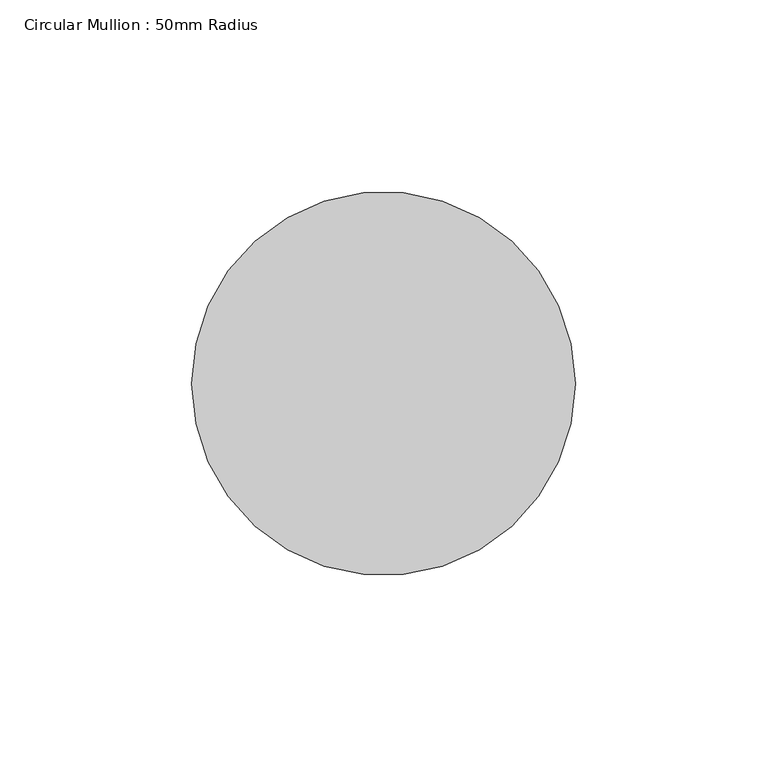
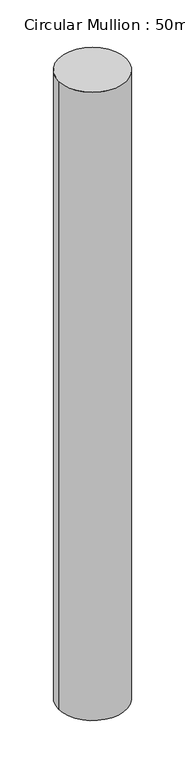
"""IFC4 building model written with IfcOpenShell, lengths in millimetres: member geometry, Circular Mullion : 50mm Radius."""

from ifc_helpers import new_model, si_unit, point, frame, origin, origin_2d, place, context, project, spatial, circle_curve, trimmed, segment, composite_curve, outline, extrude, source, transform, mapped, element, save


def circular_mullion_50mm_radius_7b3ee41a(model_context):
    return source(origin(), model_context, "Body", "SweptSolid", [
        extrude(outline(composite_curve([segment(trimmed(circle_curve(origin_2d(), 50.0), [point((50.0, 0.0))], [point((-50.0, 0.0))], False, "CARTESIAN"), True, "CONTINUOUS"), segment(trimmed(circle_curve(origin_2d(), 50.0), [point((-50.0, 0.0))], [point((50.0, 0.0))], False, "CARTESIAN"), True, "CONTINUOUS")], self_intersect=False)), frame((0.0, 0.0, -979.0567318), z_axis=(0.0, 0.0, 1.0), x_axis=(1.0, 0.0, 0.0)), (0.0, 0.0, 1.0), 979.0567318),
    ])


if __name__ == "__main__":
    model = new_model("IFC4")
    model_context = context("Model", 3, world=origin())
    ifc_project = project(units=[si_unit("LENGTHUNIT", "METRE", prefix="MILLI")], contexts=[model_context])
    site = spatial("IfcSite", under=ifc_project)
    building = spatial("IfcBuilding", under=site)
    placement = place(None, origin())
    circular_mullion_50mm_radius_shape = circular_mullion_50mm_radius_7b3ee41a(model_context)
    element("IfcMember", 1, ObjectType="Circular Mullion : 50mm Radius", at=placement, inside=building, context=model_context, shape_type="MappedRepresentation", body=[
        mapped(circular_mullion_50mm_radius_shape, transform((0.0, 0.0, 0.0), x_axis=(1.0, 0.0, 0.0), y_axis=(0.0, 1.0, 0.0), z_axis=(0.0, 0.0, 1.0))),
    ])
    save(model, "model.ifc")

# Revit data of these elements
# Type "Circular Mullion : 50mm Radius"
#   built-in parameter 1007350 = 0.164042 (stored number, unit not read)
# Element 1 (IfcMember, "Circular Mullion : 50mm Radius")
#   Materials on its faces: "Aluminium"
# Materials
#   "Aluminium": class "Metal", colour RGB 247 247 247, transparency 0, Description = "Aluminium 6061", Cost = 0
